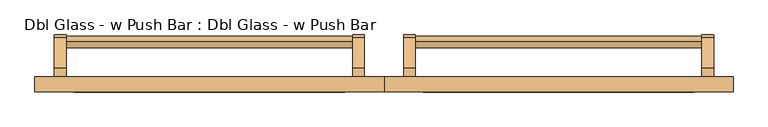
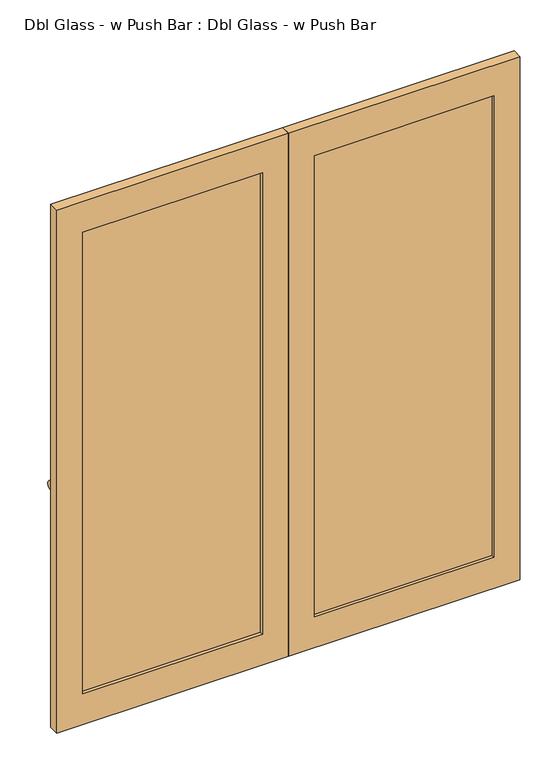
"""IFC4 building model written with IfcOpenShell, lengths in millimetres: door geometry, Dbl Glass - w Push Bar : Dbl Glass - w Push Bar."""

from ifc_helpers import new_model, si_unit, point, frame, frame_2d, origin, place, context, project, spatial, polyline, circle_curve, trimmed, segment, composite_curve, outline, extrude, source, transform, mapped, element, save


def dbl_glass_w_push_bar_dbl_glass_w_push_bar_b5e52d6e(model_context):
    return source(origin(), model_context, "Body", "SweptSolid", [
        extrude(outline(composite_curve([segment(trimmed(circle_curve(frame_2d((65.0203019, 909.5721086)), 15.0), [point((65.0203019, 924.5721086))], [point((65.0203019, 894.5721086))], False, "CARTESIAN"), True, "CONTINUOUS"), segment(trimmed(circle_curve(frame_2d((65.0203019, 909.5721086)), 15.0), [point((65.0203019, 894.5721086))], [point((65.0203019, 924.5721086))], False, "CARTESIAN"), True, "CONTINUOUS")], self_intersect=False)), frame((80.0, 0.0, 0.0), z_axis=(1.0, 0.0, 0.0), x_axis=(0.0, 1.0, 0.0)), (0.0, 0.0, 1.0), 731.0),
        extrude(outline(composite_curve([segment(polyline([(-0.1563269, 1000.0), (77.6459332, 922.19774)]), True, "CONTINUOUS"), segment(trimmed(circle_curve(frame_2d((65.0203019, 909.5721086)), 17.8553391), [point((77.6459332, 922.19774))], [point((52.3946705, 896.9464773))], False, "CARTESIAN"), True, "CONTINUOUS"), segment(polyline([(52.3946705, 896.9464773), (14.3411478, 935.0), (-24.035259, 935.0), (-24.035259, 1000.0), (-0.1563269, 1000.0)]), True, "CONTINUOUS")], self_intersect=False)), frame((811.0, 0.0, 0.0), z_axis=(1.0, 0.0, 0.0), x_axis=(0.0, 1.0, 0.0)), (0.0, 0.0, 1.0), 30.0),
        extrude(outline(composite_curve([segment(polyline([(-0.1563269, 1000.0), (77.6459332, 922.19774)]), True, "CONTINUOUS"), segment(trimmed(circle_curve(frame_2d((65.0203019, 909.5721086)), 17.8553391), [point((77.6459332, 922.19774))], [point((52.3946705, 896.9464773))], False, "CARTESIAN"), True, "CONTINUOUS"), segment(polyline([(52.3946705, 896.9464773), (14.3411478, 935.0), (-24.035259, 935.0), (-24.035259, 1000.0), (-0.1563269, 1000.0)]), True, "CONTINUOUS")], self_intersect=False)), frame((50.0, 0.0, 0.0), z_axis=(1.0, 0.0, 0.0), x_axis=(0.0, 1.0, 0.0)), (0.0, 0.0, 1.0), 30.0),
        extrude(outline(composite_curve([segment(trimmed(circle_curve(frame_2d((65.0203019, 909.5721086)), 15.0), [point((65.0203019, 924.5721086))], [point((65.0203019, 894.5721086))], False, "CARTESIAN"), True, "CONTINUOUS"), segment(trimmed(circle_curve(frame_2d((65.0203019, 909.5721086)), 15.0), [point((65.0203019, 894.5721086))], [point((65.0203019, 924.5721086))], False, "CARTESIAN"), True, "CONTINUOUS")], self_intersect=False)), frame((-811.0, 0.0, 0.0), z_axis=(1.0, 0.0, 0.0), x_axis=(0.0, 1.0, 0.0)), (0.0, 0.0, 1.0), 731.0),
        extrude(outline(composite_curve([segment(polyline([(-0.1563269, 1000.0), (77.6459332, 922.19774)]), True, "CONTINUOUS"), segment(trimmed(circle_curve(frame_2d((65.0203019, 909.5721086)), 17.8553391), [point((77.6459332, 922.19774))], [point((52.3946705, 896.9464773))], False, "CARTESIAN"), True, "CONTINUOUS"), segment(polyline([(52.3946705, 896.9464773), (14.3411478, 935.0), (-24.035259, 935.0), (-24.035259, 1000.0), (-0.1563269, 1000.0)]), True, "CONTINUOUS")], self_intersect=False)), frame((-80.0, 0.0, 0.0), z_axis=(1.0, 0.0, 0.0), x_axis=(0.0, 1.0, 0.0)), (0.0, 0.0, 1.0), 30.0),
        extrude(outline(composite_curve([segment(polyline([(-0.1563269, 1000.0), (77.6459332, 922.19774)]), True, "CONTINUOUS"), segment(trimmed(circle_curve(frame_2d((65.0203019, 909.5721086)), 17.8553391), [point((77.6459332, 922.19774))], [point((52.3946705, 896.9464773))], False, "CARTESIAN"), True, "CONTINUOUS"), segment(polyline([(52.3946705, 896.9464773), (14.3411478, 935.0), (-24.035259, 935.0), (-24.035259, 1000.0), (-0.1563269, 1000.0)]), True, "CONTINUOUS")], self_intersect=False)), frame((-841.0, 0.0, 0.0), z_axis=(1.0, 0.0, 0.0), x_axis=(0.0, 1.0, 0.0)), (0.0, 0.0, 1.0), 30.0),
        extrude(outline(polyline([(2125.0, -891.0), (0.0, -891.0), (0.0, 0.0), (2125.0, 0.0), (2125.0, -891.0)]), holes=[polyline([(2000.0, -791.0), (2000.0, -100.0), (125.0, -100.0), (125.0, -791.0), (2000.0, -791.0)])]), frame((0.0, -62.5788556, 0.0), z_axis=(0.0, 1.0, 0.0), x_axis=(0.0, 0.0, 1.0)), (0.0, 0.0, 1.0), 38.5435966),
        extrude(outline(polyline([(2125.0, 0.0), (0.0, 0.0), (0.0, 891.0), (2125.0, 891.0), (2125.0, 0.0)]), holes=[polyline([(2000.0, 100.0), (2000.0, 791.0), (125.0, 791.0), (125.0, 100.0), (2000.0, 100.0)])]), frame((0.0, -62.5788556, 0.0), z_axis=(0.0, 1.0, 0.0), x_axis=(0.0, 0.0, 1.0)), (0.0, 0.0, 1.0), 38.5435966),
        extrude(outline(polyline([(-100.0, -38.0), (-100.0, -50.0), (-791.0, -50.0), (-791.0, -38.0), (-100.0, -38.0)])), frame((0.0, 0.0, 125.0), z_axis=(0.0, 0.0, 1.0), x_axis=(1.0, 0.0, 0.0)), (0.0, 0.0, 1.0), 1875.0),
        extrude(outline(polyline([(791.0, -38.0), (791.0, -50.0), (100.0, -50.0), (100.0, -38.0), (791.0, -38.0)])), frame((0.0, 0.0, 125.0), z_axis=(0.0, 0.0, 1.0), x_axis=(1.0, 0.0, 0.0)), (0.0, 0.0, 1.0), 1875.0),
    ])


if __name__ == "__main__":
    model = new_model("IFC4")
    model_context = context("Model", 3, world=origin())
    ifc_project = project(units=[si_unit("LENGTHUNIT", "METRE", prefix="MILLI")], contexts=[model_context])
    site = spatial("IfcSite", under=ifc_project)
    building = spatial("IfcBuilding", under=site)
    placement = place(None, origin())
    dbl_glass_w_push_bar_dbl_glass_w_push_bar_shape = dbl_glass_w_push_bar_dbl_glass_w_push_bar_b5e52d6e(model_context)
    element("IfcDoor", 1, ObjectType="Dbl Glass - w Push Bar : Dbl Glass - w Push Bar", at=placement, inside=building, context=model_context, shape_type="MappedRepresentation", body=[
        mapped(dbl_glass_w_push_bar_dbl_glass_w_push_bar_shape, transform((0.0, 0.0, 0.0), x_axis=(1.0, 0.0, 0.0), y_axis=(0.0, 1.0, 0.0), z_axis=(0.0, 0.0, 1.0))),
    ])
    save(model, "model.ifc")

# Revit data of these elements
# Type "Dbl Glass - w Push Bar : Dbl Glass - w Push Bar"
#   Description = "Curtain Wall Door"
#   Type Mark = "55"
#   Construction Type Id = "GSP4R"
#   Analytic Construction = "1/8 in Pilkington single glazing"
#   Visual Light Transmittance = 0.9
#   TopRail = 125 mm
#   Solar Heat Gain Coefficient = 0.78
#   Offset = 50 mm
#   MuntinRail = 100 mm
#   LockRail = 100 mm
#   Heat Transfer Coefficient (U) = 3.6886 W/(m²·K)
#   Handle Z Distance = 1000 mm
#   Handle X Offset = 65 mm
#   Glass Thickness = 12 mm
#   BottomRail = 125 mm
#   Define Thermal Properties by = 1
#   Material Ironmongery = Metal - Aluminum
#   Material Door = Metal - Aluminum
#   Material Glass = Glass
#   Function = (empty or 0)
# Element 1 (IfcDoor, "Dbl Glass - w Push Bar : Dbl Glass - w Push Bar")
#   Materials on its faces: "Metal - Aluminum", "Glass"
# Materials
#   "Metal - Aluminum": class "Metal", colour RGB 247 247 247, transparency 0
#   "Glass": class "Glass", colour RGB 0 128 192, transparency 0.9, Description = "Soda Lime Glass", Cost = 0
